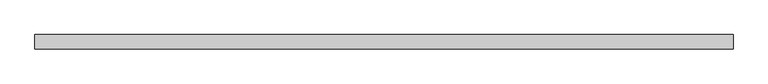
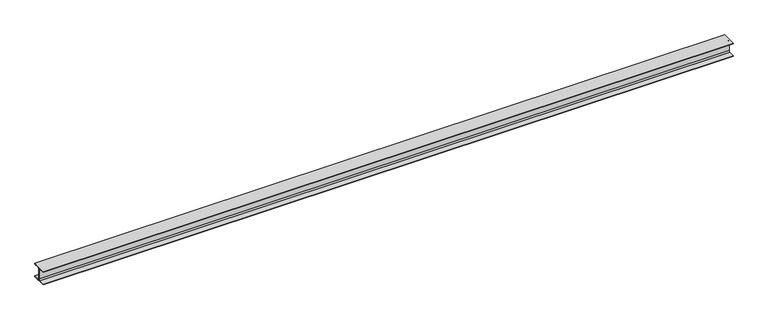
"""IFC4 building model written with IfcOpenShell, lengths in millimetres: beam geometry, NLRS_28_SF_LIB_stalen ligger HEB-AV-CWV-MMBS-SRP_gen_rsf : stalen ligger_gen__HEB 260."""

from ifc_helpers import new_model, si_unit, point, frame, frame_2d, origin, place, context, project, spatial, polyline, circle_curve, trimmed, segment, composite_curve, outline, extrude, source, transform, mapped, element, save


def beam_0ced8335(model_context):
    return source(origin(), model_context, "Body", "SweptSolid", [
        extrude(outline(composite_curve([segment(polyline([(130.0, 112.5), (29.0, 112.5)]), True, "CONTINUOUS"), segment(trimmed(circle_curve(frame_2d((29.0, 88.5)), 24.0), [point((29.0, 112.5))], [point((5.0, 88.5))], True, "CARTESIAN"), True, "CONTINUOUS"), segment(polyline([(5.0, 88.5), (5.0, -88.5)]), True, "CONTINUOUS"), segment(trimmed(circle_curve(frame_2d((29.0, -88.5)), 24.0), [point((5.0, -88.5))], [point((29.0, -112.5))], True, "CARTESIAN"), True, "CONTINUOUS"), segment(polyline([(29.0, -112.5), (130.0, -112.5), (130.0, -130.0), (-130.0, -130.0), (-130.0, -112.5), (-29.0, -112.5)]), True, "CONTINUOUS"), segment(trimmed(circle_curve(frame_2d((-29.0, -88.5)), 24.0), [point((-29.0, -112.5))], [point((-5.0, -88.5))], True, "CARTESIAN"), True, "CONTINUOUS"), segment(polyline([(-5.0, -88.5), (-5.0, 88.5)]), True, "CONTINUOUS"), segment(trimmed(circle_curve(frame_2d((-29.0, 88.5)), 24.0), [point((-5.0, 88.5))], [point((-29.0, 112.5))], True, "CARTESIAN"), True, "CONTINUOUS"), segment(polyline([(-29.0, 112.5), (-130.0, 112.5), (-130.0, 130.0), (130.0, 130.0), (130.0, 112.5)]), True, "CONTINUOUS")], self_intersect=False)), frame((-6318.75, 0.0, 0.0), z_axis=(1.0, 0.0, 0.0), x_axis=(0.0, 1.0, 0.0)), (0.0, 0.0, 1.0), 12637.5),
    ])


if __name__ == "__main__":
    model = new_model("IFC4")
    model_context = context("Model", 3, world=origin())
    ifc_project = project(units=[si_unit("LENGTHUNIT", "METRE", prefix="MILLI")], contexts=[model_context])
    site = spatial("IfcSite", under=ifc_project)
    building = spatial("IfcBuilding", under=site)
    placement = place(None, origin())
    beam_shape = beam_0ced8335(model_context)
    element("IfcBeam", 1, ObjectType="NLRS_28_SF_LIB_stalen ligger HEB-AV-CWV-MMBS-SRP_gen_rsf : stalen ligger_gen__HEB 260", at=placement, inside=building, context=model_context, shape_type="MappedRepresentation", body=[
        mapped(beam_shape, transform((0.0, 0.0, 0.0), x_axis=(1.0, 0.0, 0.0), y_axis=(0.0, 1.0, 0.0), z_axis=(0.0, 0.0, 1.0))),
    ])
    save(model, "model.ifc")

# Revit data of these elements
# Type "NLRS_28_SF_LIB_stalen ligger HEB-AV-CWV-MMBS-SRP_gen_rsf : stalen ligger_gen__HEB 260"
#   Export Type to IFC As = "IfcBeamType"
#   Type IfcGUID = "0zo1UjqZ91lRsfCKsOOa5a"
#   Type Comments = "HEB260"
#   Model = " "
#   Manufacturer = " "
#   Fire Rating = " "
#   Description = "stalen ligger HEB260"
#   Assembly Code = "28.11"
#   ra = 24 mm
#   vz = 130 mm
#   vy = 130 mm
#   vpz = 130 mm
#   vpy = 130 mm
#   NLRS_C_lengte [instance default] = 1500 mm
#   Length [instance default] = 1500 mm
#   bf = 260 mm
#   d = 260 mm
#   tf = 17.5 mm
#   tw = 10 mm
#   Structural Material = NLRS_h2_staal_gen_rsf
#   Keynote = ""
# Element 1 (IfcBeam, "NLRS_28_SF_LIB_stalen ligger HEB-AV-CWV-MMBS-SRP_gen_rsf : stalen ligger_gen__HEB 260")
#   NLRS_C_lengte = 12637.5 mm
#   Materials on its faces: "NLRS_h2_staal_gen_rsf"
# Materials
#   "NLRS_h2_staal_gen_rsf": class "H - Metaal", colour RGB 189 187 185, transparency 0, Keynote = "h2", Manufacturer = "Revit Standards Foundation", URL = "www.revitstandards.org", Description = "staal", Cost = 0
